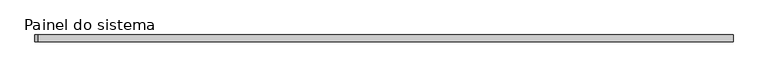
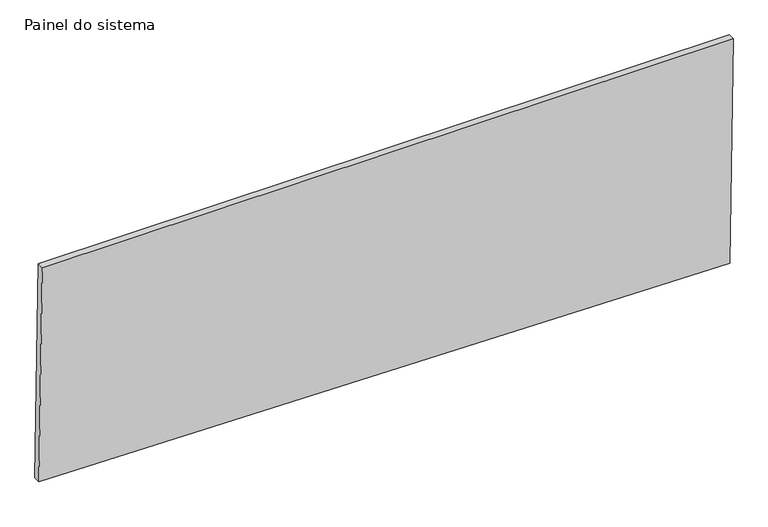
"""IFC4 building model written with IfcOpenShell, lengths in millimetres: plate geometry, Painel do sistema : Envidraçado."""

from ifc_helpers import new_model, si_unit, frame, origin, place, context, project, spatial, polyline, outline, extrude, source, transform, mapped, element, save


def painel_do_sistema_8d8d8803(model_context):
    return source(origin(), model_context, "Body", "SweptSolid", [
        extrude(outline(polyline([(37.9368749, -1267.6464289), (0.0, 1254.6972339), (860.9649598, 1267.6464289), (860.9649598, -1255.2678169), (37.9368749, -1267.6464289)])), frame((0.0, 24.5, 0.0), z_axis=(0.0, 1.0, 0.0), x_axis=(0.0, 0.0, 1.0)), (0.0, 0.0, 1.0), 25.0),
    ])


if __name__ == "__main__":
    model = new_model("IFC4")
    model_context = context("Model", 3, world=origin())
    ifc_project = project(units=[si_unit("LENGTHUNIT", "METRE", prefix="MILLI")], contexts=[model_context])
    site = spatial("IfcSite", under=ifc_project)
    building = spatial("IfcBuilding", under=site)
    placement = place(None, origin())
    painel_do_sistema_shape = painel_do_sistema_8d8d8803(model_context)
    element("IfcPlate", 1, ObjectType="Painel do sistema : Envidraçado", at=placement, inside=building, context=model_context, shape_type="MappedRepresentation", body=[
        mapped(painel_do_sistema_shape, transform((0.0, 0.0, 0.0), x_axis=(1.0, 0.0, 0.0), y_axis=(0.0, 1.0, 0.0), z_axis=(0.0, 0.0, 1.0))),
    ])
    save(model, "model.ifc")

# Revit data of these elements
# Type "Painel do sistema : Envidraçado"
#   Construction Type Id = "GSP4R"
#   Analytic Construction = "Vidraça única Pilkington 1/8 pol"
#   Visual Light Transmittance = 0.9
#   Solar Heat Gain Coefficient = 0.86
#   Heat Transfer Coefficient (U) = 6.7069 W/(m²·K)
# Element 1 (IfcPlate, "Painel do sistema : Envidraçado")
#   Materials on its faces: "Vidro"
# Materials
#   "Vidro": class "Vidro", colour RGB 0 128 192, transparency 0.9, Description = "Vidro de sílica", Cost = 0
